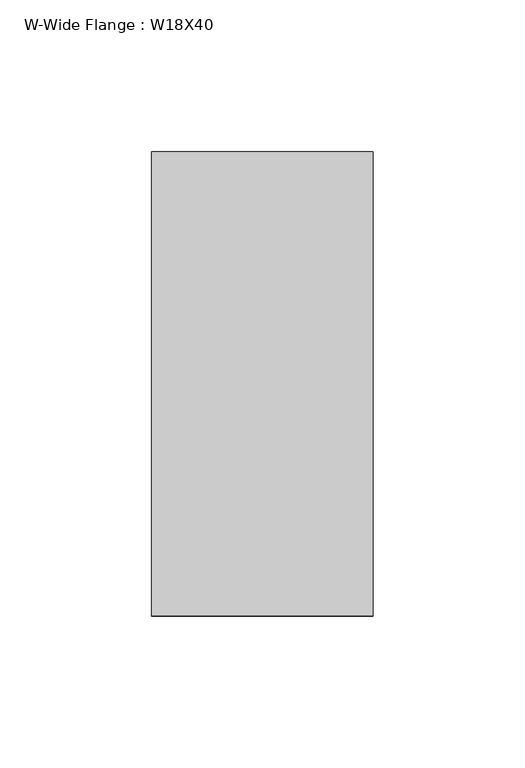
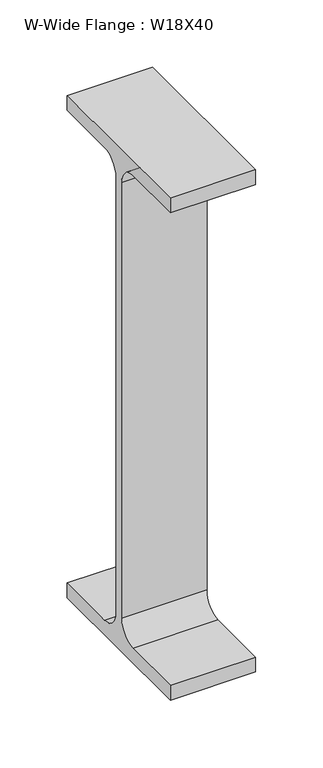
"""IFC4 building model written with IfcOpenShell, lengths in millimetres: beam geometry, W-Wide Flange : W18X40."""

import ifcopenshell
import ifcopenshell.guid

model = None  # the IFC model being written
_history = None  # IfcOwnerHistory: only IFC2X3 demands one
_inside = {}  # id of a spatial element -> (the spatial element, [elements in it])
_under = {}  # id of a project, library or spatial element -> (it, [spatial elements below it])
_declared = {}  # id of a project -> (the project, [libraries it declares])
_typed = {}  # id of a type object -> (the type object, [elements of that type])
_made_of = {}  # id of a material, layer set ... -> (it, [elements and type objects made of it])


def new_model(schema):
    """Start an empty IFC model of exactly this schema.

    Asked for "IFC4X3", IfcOpenShell would pick the latest addendum, in which some entities
    have other attributes; the version numbers below select the first issue.
    IFC2X3 requires an IfcOwnerHistory on every rooted entity: one is made here for all.
    """
    global model, _history
    if schema == "IFC4X3":
        model = ifcopenshell.file(schema_version=(4, 3, 0, 0))
    else:
        model = ifcopenshell.file(schema=schema)
    _inside.clear()
    _under.clear()
    _declared.clear()
    _typed.clear()
    _made_of.clear()
    _history = None
    if model.schema == "IFC2X3":
        org = make("IfcOrganization", Name="unknown")
        user = make(
            "IfcPersonAndOrganization",
            ThePerson=make("IfcPerson", FamilyName="unknown"),
            TheOrganization=org,
        )
        app = make(
            "IfcApplication",
            ApplicationDeveloper=org,
            Version="unknown",
            ApplicationFullName="unknown",
            ApplicationIdentifier="unknown",
        )
        _history = make(
            "IfcOwnerHistory",
            OwningUser=user,
            OwningApplication=app,
            ChangeAction="ADDED",
            CreationDate=0,
        )
    return model


def make(cls, **values):
    """One entity of the class cls with the attributes given. An attribute that is None is left unset."""
    return model.create_entity(
        cls, **{name: value for name, value in values.items() if value is not None}
    )


def rooted(cls, **values):
    """An entity with a GlobalId (a new one), such as an element, a storey or a relation."""
    return make(cls, GlobalId=ifcopenshell.guid.new(), OwnerHistory=_history, **values)


def si_unit(unit_type, name, prefix=None):
    """IfcSIUnit, for example si_unit("LENGTHUNIT", "METRE", prefix="MILLI")."""
    return make("IfcSIUnit", UnitType=unit_type, Prefix=prefix, Name=name)


def assignment(units):
    """IfcUnitAssignment: the units of a project."""
    return None if units is None else make("IfcUnitAssignment", Units=units)


def point(xyz):
    """IfcCartesianPoint."""
    return None if xyz is None else make("IfcCartesianPoint", Coordinates=xyz)


def direction(xyz):
    """IfcDirection."""
    return None if xyz is None else make("IfcDirection", DirectionRatios=xyz)


def frame(location, z_axis=None, x_axis=None):
    """IfcAxis2Placement3D, a coordinate frame: its origin and axes. An axis left out is left unset."""
    return make(
        "IfcAxis2Placement3D",
        Location=point(location),
        Axis=direction(z_axis),
        RefDirection=direction(x_axis),
    )


def frame_2d(location, x_axis=None):
    """IfcAxis2Placement2D, a coordinate frame in the plane: its origin and x axis."""
    return make(
        "IfcAxis2Placement2D", Location=point(location), RefDirection=direction(x_axis)
    )


def origin():
    """The frame at (0, 0, 0) with its axes left unset."""
    return frame((0.0, 0.0, 0.0))


def place(relative_to, where):
    """IfcLocalPlacement: puts the frame where relative to a parent placement (None: the world)."""
    return make(
        "IfcLocalPlacement", PlacementRelTo=relative_to, RelativePlacement=where
    )


def context(
    kind, dimensions, precision=None, world=None, true_north=None, identifier=None
):
    """IfcGeometricRepresentationContext, for example the 3D "Model" context."""
    return make(
        "IfcGeometricRepresentationContext",
        ContextIdentifier=identifier,
        ContextType=kind,
        CoordinateSpaceDimension=dimensions,
        Precision=precision,
        WorldCoordinateSystem=world,
        TrueNorth=true_north,
    )


def project(units=None, contexts=None):
    """IfcProject with its units and contexts."""
    return rooted(
        "IfcProject",
        Name="project",
        RepresentationContexts=contexts,
        UnitsInContext=assignment(units),
    )


def spatial(cls, under=None, at=None, **own):
    """A site, building, storey or space (cls), placed at a placement, below another one or the project."""
    s = rooted(cls, ObjectPlacement=at, **own)
    if under is not None:
        _under.setdefault(under.id(), (under, []))[1].append(s)
    return s


def polyline(points):
    """IfcPolyline through the points."""
    return make("IfcPolyline", Points=[point(p) for p in points])


def circle_curve(where, radius):
    """IfcCircle in the frame where."""
    return make("IfcCircle", Position=where, Radius=radius)


def trimmed(basis, trim1, trim2, sense, master):
    """IfcTrimmedCurve: the piece of a basis curve between two trims."""
    return make(
        "IfcTrimmedCurve",
        BasisCurve=basis,
        Trim1=trim1,
        Trim2=trim2,
        SenseAgreement=sense,
        MasterRepresentation=master,
    )


def segment(curve, same_sense, transition):
    """IfcCompositeCurveSegment."""
    return make(
        "IfcCompositeCurveSegment",
        Transition=transition,
        SameSense=same_sense,
        ParentCurve=curve,
    )


def composite_curve(segments, self_intersect=None):
    """IfcCompositeCurve: segments joined end to end."""
    return make("IfcCompositeCurve", Segments=segments, SelfIntersect=self_intersect)


def outline(outer, holes=None, kind="AREA"):
    """IfcArbitraryClosedProfileDef: a profile drawn as a closed curve; with holes, ...WithVoids."""
    if holes is None:
        return make("IfcArbitraryClosedProfileDef", ProfileType=kind, OuterCurve=outer)
    return make(
        "IfcArbitraryProfileDefWithVoids",
        ProfileType=kind,
        OuterCurve=outer,
        InnerCurves=holes,
    )


def extrude(swept, where, along, depth):
    """IfcExtrudedAreaSolid: the profile swept, set in the frame where, extruded along a direction by depth."""
    return make(
        "IfcExtrudedAreaSolid",
        SweptArea=swept,
        Position=where,
        ExtrudedDirection=direction(along),
        Depth=depth,
    )


def shape(context_of_items, identifier, shape_type, items):
    """IfcShapeRepresentation: the items that make up one representation, for example the "Body"."""
    return make(
        "IfcShapeRepresentation",
        ContextOfItems=context_of_items,
        RepresentationIdentifier=identifier,
        RepresentationType=shape_type,
        Items=items,
    )


def source(mapping_origin, context_of_items, identifier, shape_type, items):
    """IfcRepresentationMap: a shape defined once, which mapped items show again and again."""
    return make(
        "IfcRepresentationMap",
        MappingOrigin=mapping_origin,
        MappedRepresentation=shape(context_of_items, identifier, shape_type, items),
    )


def transform(
    local_origin,
    x_axis=None,
    y_axis=None,
    z_axis=None,
    scale=None,
    scale2=None,
    scale3=None,
    uniform=True,
):
    """IfcCartesianTransformationOperator3D, or its non-uniform kind. x_axis, y_axis, z_axis: its Axis1, 2, 3."""
    if uniform:
        return make(
            "IfcCartesianTransformationOperator3D",
            Axis1=direction(x_axis),
            Axis2=direction(y_axis),
            LocalOrigin=point(local_origin),
            Scale=scale,
            Axis3=direction(z_axis),
        )
    return make(
        "IfcCartesianTransformationOperator3DnonUniform",
        Axis1=direction(x_axis),
        Axis2=direction(y_axis),
        LocalOrigin=point(local_origin),
        Scale=scale,
        Axis3=direction(z_axis),
        Scale2=scale2,
        Scale3=scale3,
    )


def mapped(mapping_source, mapping_target):
    """IfcMappedItem: shows the shape of a source again, moved by a transform."""
    return make(
        "IfcMappedItem", MappingSource=mapping_source, MappingTarget=mapping_target
    )


def made_of(thing, what):
    """Note that an element or type object is made of a material, layer set ...; save() writes the relation."""
    if what is not None:
        _made_of.setdefault(what.id(), (what, []))[1].append(thing)
    return thing


def element(
    cls,
    number,
    at=None,
    inside=None,
    cuts=None,
    type_object=None,
    material=None,
    context=None,
    identifier="Body",
    shape_type=None,
    held_by="IfcProductDefinitionShape",
    body=None,
    shapes=None,
    **own,
):
    """One element of the class cls, such as IfcWall. Its Tag is "e" and its number.

    at: its placement. inside: the storey or other place that contains it. cuts: it is an
    opening in that element (IfcRelVoidsElement). A single representation is given by context,
    identifier, shape_type and body (its items); several are given by shapes. held_by: the class
    of the entity that holds the representations. save() writes the other relations.
    """
    e = rooted(cls, Tag="e%d" % number, ObjectPlacement=at, **own)
    if body is not None:
        shapes = [shape(context, identifier, shape_type, body)]
    if shapes is not None:
        e.Representation = make(held_by, Representations=shapes)
    if inside is not None:
        _inside.setdefault(inside.id(), (inside, []))[1].append(e)
    if cuts is not None:
        rooted(
            "IfcRelVoidsElement", RelatingBuildingElement=cuts, RelatedOpeningElement=e
        )
    if type_object is not None:
        _typed.setdefault(type_object.id(), (type_object, []))[1].append(e)
    return made_of(e, material)


def aggregate(whole, parts):
    """IfcRelAggregates: a whole, such as a stair, and the parts it consists of."""
    return rooted("IfcRelAggregates", RelatingObject=whole, RelatedObjects=parts)


def save(model, path):
    """Write the relations noted so far, then the file.

    IfcRelAggregates (storeys below a building ...), IfcRelContainedInSpatialStructure (elements
    in a storey), IfcRelDefinesByType, IfcRelAssociatesMaterial and IfcRelDeclares: one each for
    every whole, place, type object, material and project.
    """
    for whole, parts in _under.values():
        aggregate(whole, parts)
    for where, things in _inside.values():
        rooted(
            "IfcRelContainedInSpatialStructure",
            RelatedElements=things,
            RelatingStructure=where,
        )
    for kind, things in _typed.values():
        rooted("IfcRelDefinesByType", RelatedObjects=things, RelatingType=kind)
    for what, things in _made_of.values():
        rooted("IfcRelAssociatesMaterial", RelatedObjects=things, RelatingMaterial=what)
    for by, libraries in _declared.values():
        rooted("IfcRelDeclares", RelatingContext=by, RelatedDefinitions=libraries)
    model.write(path)


def w_wide_flange_w18x40_6c12524d(model_context):
    return source(origin(), model_context, "Body", "SweptSolid", [
        extrude(outline(composite_curve([segment(polyline([(-76.454, -213.995), (-20.828, -213.995)]), True, "CONTINUOUS"), segment(trimmed(circle_curve(frame_2d((-20.828, -197.1675)), 16.8275), [point((-20.828, -213.995))], [point((-4.0005, -197.1675))], True, "CARTESIAN"), True, "CONTINUOUS"), segment(polyline([(-4.0005, -197.1675), (-4.0005, 197.1675)]), True, "CONTINUOUS"), segment(trimmed(circle_curve(frame_2d((-20.828, 197.1675)), 16.8275), [point((-4.0005, 197.1675))], [point((-20.828, 213.995))], True, "CARTESIAN"), True, "CONTINUOUS"), segment(polyline([(-20.828, 213.995), (-76.454, 213.995), (-76.454, 227.33), (76.454, 227.33), (76.454, 213.995), (20.828, 213.995)]), True, "CONTINUOUS"), segment(trimmed(circle_curve(frame_2d((20.828, 197.1675)), 16.8275), [point((20.828, 213.995))], [point((4.0005, 197.1675))], True, "CARTESIAN"), True, "CONTINUOUS"), segment(polyline([(4.0005, 197.1675), (4.0005, -197.1675)]), True, "CONTINUOUS"), segment(trimmed(circle_curve(frame_2d((20.828, -197.1675)), 16.8275), [point((4.0005, -197.1675))], [point((20.828, -213.995))], True, "CARTESIAN"), True, "CONTINUOUS"), segment(polyline([(20.828, -213.995), (76.454, -213.995), (76.454, -227.33), (-76.454, -227.33), (-76.454, -213.995)]), True, "CONTINUOUS")], self_intersect=False)), frame((-30.95625, 0.0, 0.0), z_axis=(1.0, 0.0, 0.0), x_axis=(0.0, 1.0, 0.0)), (0.0, 0.0, 1.0), 73.025),
    ])


if __name__ == "__main__":
    model = new_model("IFC4")
    model_context = context("Model", 3, world=origin())
    ifc_project = project(units=[si_unit("LENGTHUNIT", "METRE", prefix="MILLI")], contexts=[model_context])
    site = spatial("IfcSite", under=ifc_project)
    building = spatial("IfcBuilding", under=site)
    placement = place(None, origin())
    w_wide_flange_w18x40_shape = w_wide_flange_w18x40_6c12524d(model_context)
    element("IfcBeam", 1, ObjectType="W-Wide Flange : W18X40", at=placement, inside=building, context=model_context, shape_type="MappedRepresentation", body=[
        mapped(w_wide_flange_w18x40_shape, transform((0.0, 0.0, 0.0), x_axis=(1.0, 0.0, 0.0), y_axis=(0.0, 1.0, 0.0), z_axis=(0.0, 0.0, 1.0))),
    ])
    save(model, "model.ifc")

# Revit data of these elements
# Type "W-Wide Flange : W18X40"
#   Assembly Code = "B10"
#   W = 40
#   Length [instance default] = 5' - 0"
#   bf = 0' - 6.02"
#   d = 1' - 5.9"
#   k = 0' - 1 3/16"
#   k2 = 0' - 0.6625"
#   tf = 0' - 0.525"
#   tw = 0' - 0.315"
#   A = 0.0819444 SF
#   Structural Material [instance default] = Steel ASTM A992
# Element 1 (IfcBeam, "W-Wide Flange : W18X40")
#   Materials on its faces: "Steel ASTM A992"
# Materials
#   "Steel ASTM A992": class "Metal", colour RGB 199 199 199, transparency 0, Description = "Structural steel 50ksi", Cost = 0
